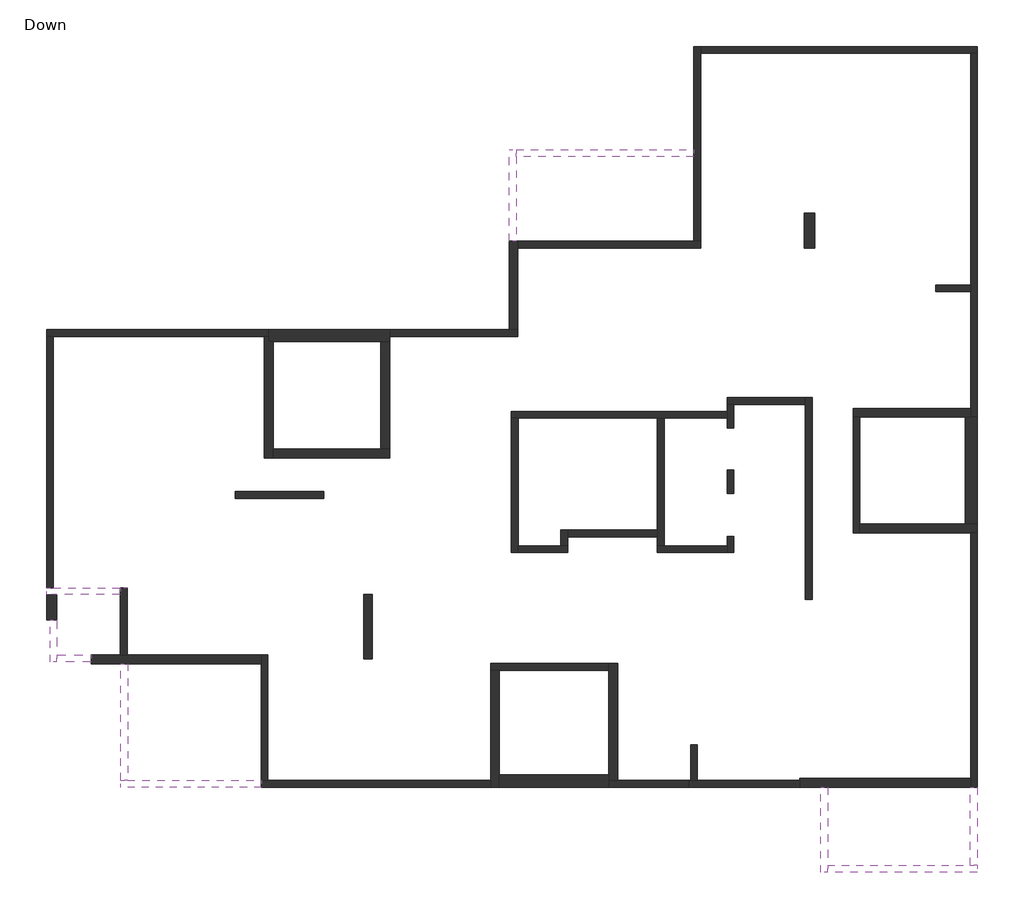
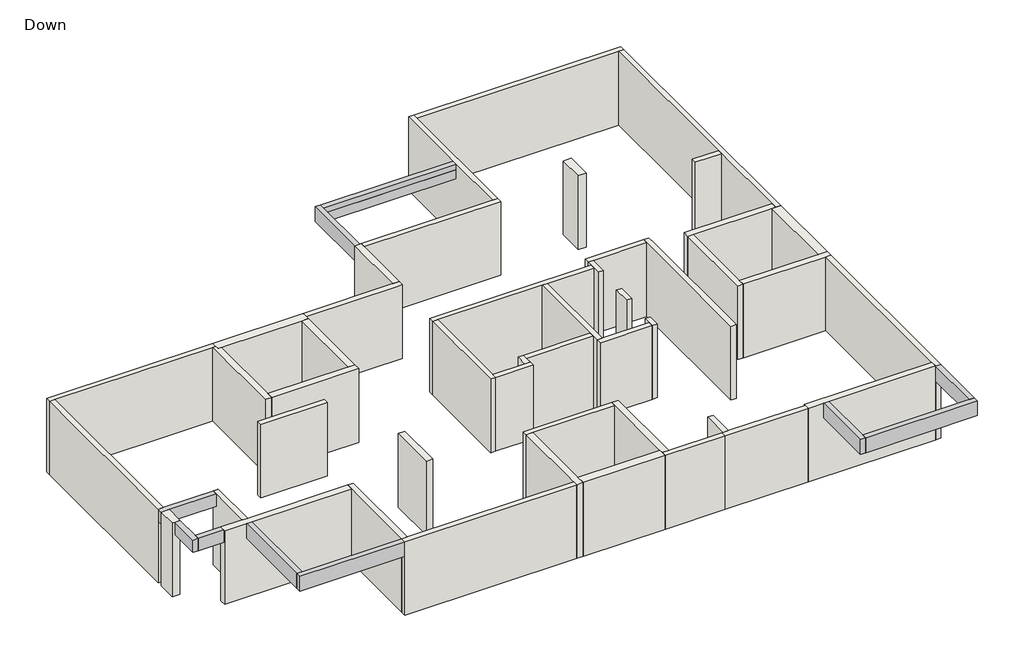
# One storey: 46 walls, 10 beams.
# Revit data of these elements (continued)
# Element 19 (IfcWall, "20") (continued)
#   SOFiSTiK_AMG_Scheduled = yes
#   SOFiSTiK_AMG_Adjusted = yes
#   Phase Created = New Construction
#   Base Constraint = Down
#   Top Constraint = Typical Floor
#   Materials on its faces: "Concrete"
# Element 20 (IfcWall, "20")
#   Comments = ""
#   Mark = "W10"
#   SOFiSTiK_EdgeZones = "W10"
#   SOFiSTiK_AMG_Comments = ""
#   Top Offset = 0 cm
#   Base Offset = 0 cm
#   wall height = 300 cm
#   SOFiSTiK_AMG_Scheduled = yes
#   SOFiSTiK_AMG_Adjusted = yes
#   Phase Created = New Construction
#   Base Constraint = Down
#   Top Constraint = Typical Floor
#   Materials on its faces: "Concrete"
# Element 21 (IfcWall, "20")
#   Comments = ""
#   Mark = "W11"
#   SOFiSTiK_EdgeZones = "W11"
#   SOFiSTiK_AMG_Comments = ""
#   Top Offset = 0 cm
#   Base Offset = 0 cm
#   wall height = 300 cm
#   SOFiSTiK_AMG_Scheduled = yes
#   SOFiSTiK_AMG_Adjusted = yes
#   Phase Created = New Construction
#   Base Constraint = Down
#   Top Constraint = Typical Floor
#   Materials on its faces: "Concrete"
# Element 22 (IfcWall, "20")
#   Comments = ""
#   Mark = "W12"
#   SOFiSTiK_EdgeZones = "W12"
#   SOFiSTiK_AMG_Comments = ""
#   Top Offset = 0 cm
#   Base Offset = 0 cm
#   wall height = 300 cm
#   SOFiSTiK_AMG_Scheduled = yes
#   SOFiSTiK_AMG_Adjusted = yes
#   Phase Created = New Construction
#   Base Constraint = Down
#   Top Constraint = Typical Floor
#   Materials on its faces: "Concrete"
# Element 23 (IfcWall, "20")
#   Comments = ""
#   Mark = "W13"
#   SOFiSTiK_EdgeZones = "W13"
#   SOFiSTiK_AMG_Comments = ""
#   Top Offset = 0 cm
#   Base Offset = 0 cm
#   wall height = 300 cm
#   SOFiSTiK_AMG_Scheduled = yes
#   SOFiSTiK_AMG_Adjusted = yes
#   Phase Created = New Construction
#   Base Constraint = Down
#   Top Constraint = Typical Floor
#   Materials on its faces: "Concrete"
# Element 24 (IfcWall, "20")
#   Comments = ""
#   Mark = "W14"
#   SOFiSTiK_EdgeZones = "W14"
#   SOFiSTiK_AMG_Comments = ""
#   Top Offset = 0 cm
#   Base Offset = 0 cm
#   wall height = 300 cm
#   SOFiSTiK_AMG_Scheduled = yes
#   SOFiSTiK_AMG_Adjusted = yes
#   Phase Created = New Construction
#   Base Constraint = Down
#   Top Constraint = Typical Floor
#   Materials on its faces: "Concrete"
# Element 25 (IfcWall, "20")
#   Comments = ""
#   Mark = "W15"
#   SOFiSTiK_EdgeZones = "W15"
#   SOFiSTiK_AMG_Comments = ""
#   Top Offset = 0 cm
#   Base Offset = 0 cm
#   wall height = 300 cm
#   SOFiSTiK_AMG_Scheduled = yes
#   SOFiSTiK_AMG_Adjusted = yes
#   Phase Created = New Construction
#   Base Constraint = Down
#   Top Constraint = Typical Floor
#   Materials on its faces: "Concrete"
# Element 26 (IfcWall, "20")
#   Comments = ""
#   Mark = "W16"
#   SOFiSTiK_EdgeZones = "W16"
#   SOFiSTiK_AMG_Comments = ""
#   Top Offset = 0 cm
#   Base Offset = 0 cm
#   wall height = 300 cm
#   SOFiSTiK_AMG_Scheduled = yes
#   SOFiSTiK_AMG_Adjusted = yes
#   Phase Created = New Construction
#   Base Constraint = Down
#   Top Constraint = Typical Floor
#   Materials on its faces: "Concrete"
# Element 27 (IfcWall, "20")
#   Comments = ""
#   Mark = "W17"
#   SOFiSTiK_EdgeZones = "W17"
#   SOFiSTiK_AMG_Comments = ""
#   Top Offset = 0 cm
#   Base Offset = 0 cm
#   wall height = 300 cm
#   SOFiSTiK_AMG_Scheduled = yes
#   SOFiSTiK_AMG_Adjusted = yes
#   Phase Created = New Construction
#   Base Constraint = Down
#   Top Constraint = Typical Floor
#   Materials on its faces: "Concrete"
# Element 28 (IfcWall, "20")
#   Comments = ""
#   Mark = "W18"
#   SOFiSTiK_EdgeZones = "W18"
#   SOFiSTiK_AMG_Comments = ""
#   Top Offset = 0 cm
#   Base Offset = 0 cm
#   wall height = 300 cm
#   SOFiSTiK_AMG_Scheduled = yes
#   SOFiSTiK_AMG_Adjusted = yes
#   Phase Created = New Construction
#   Base Constraint = Down
#   Top Constraint = Typical Floor
#   Materials on its faces: "Concrete"
# Element 29 (IfcWall, "20")
#   Comments = ""
#   Mark = "W19"
#   SOFiSTiK_EdgeZones = "W19"
#   SOFiSTiK_AMG_Comments = ""
#   Top Offset = 0 cm
#   Base Offset = 0 cm
#   wall height = 300 cm
#   SOFiSTiK_AMG_Scheduled = yes
#   SOFiSTiK_AMG_Adjusted = yes
#   Phase Created = New Construction
#   Base Constraint = Down
#   Top Constraint = Typical Floor
#   Materials on its faces: "Concrete"
# Element 30 (IfcWall, "20")
#   Comments = ""
#   Mark = "W20"
#   SOFiSTiK_EdgeZones = "W20"
#   SOFiSTiK_AMG_Comments = ""
#   Top Offset = 0 cm
#   Base Offset = 0 cm
#   wall height = 300 cm
#   SOFiSTiK_AMG_Scheduled = yes
#   SOFiSTiK_AMG_Adjusted = yes
#   Phase Created = New Construction
#   Base Constraint = Down
#   Top Constraint = Typical Floor
#   Materials on its faces: "Concrete"
# Element 31 (IfcWall, "20")
#   Comments = ""
#   Mark = "W21"
#   SOFiSTiK_EdgeZones = "W21"
#   SOFiSTiK_AMG_Comments = ""
#   Top Offset = 0 cm
#   Base Offset = 0 cm
#   wall height = 300 cm
#   SOFiSTiK_AMG_Scheduled = yes
#   SOFiSTiK_AMG_Adjusted = yes
#   Phase Created = New Construction
#   Base Constraint = Down
#   Top Constraint = Typical Floor
#   Materials on its faces: "Concrete"
# Element 32 (IfcWall, "20")
#   Comments = ""
#   Mark = "W22"
#   SOFiSTiK_EdgeZones = "W22"
#   SOFiSTiK_AMG_Comments = ""
#   Top Offset = 0 cm
#   Base Offset = 0 cm
#   wall height = 300 cm
#   SOFiSTiK_AMG_Scheduled = yes
#   SOFiSTiK_AMG_Adjusted = yes
#   Phase Created = New Construction
#   Base Constraint = Down
#   Top Constraint = Typical Floor
#   Materials on its faces: "Concrete"
# Element 33 (IfcWall, "20")
#   Comments = ""
#   Mark = "W23"
#   SOFiSTiK_EdgeZones = "W23"
#   SOFiSTiK_AMG_Comments = ""
#   Top Offset = 0 cm
#   Base Offset = 0 cm
#   wall height = 300 cm
#   SOFiSTiK_AMG_Scheduled = yes
#   SOFiSTiK_AMG_Adjusted = yes
#   Phase Created = New Construction
#   Base Constraint = Down
#   Top Constraint = Typical Floor
#   Materials on its faces: "Concrete"
# Element 34 (IfcWall, "20")
#   Comments = ""
#   Mark = "W24"
#   SOFiSTiK_EdgeZones = "W24"
#   SOFiSTiK_AMG_Comments = ""
#   Top Offset = 0 cm
#   Base Offset = 0 cm
#   wall height = 300 cm
#   SOFiSTiK_AMG_Scheduled = yes
#   SOFiSTiK_AMG_Adjusted = yes
#   Phase Created = New Construction
#   Base Constraint = Down
#   Top Constraint = Typical Floor
#   Materials on its faces: "Concrete"
# Element 35 (IfcWall, "20")
#   Comments = ""
#   Mark = "W25"
#   SOFiSTiK_EdgeZones = "W25"
#   SOFiSTiK_AMG_Comments = ""
#   Top Offset = 0 cm
#   Base Offset = 0 cm
#   wall height = 300 cm
#   SOFiSTiK_AMG_Scheduled = yes
#   SOFiSTiK_AMG_Adjusted = yes
#   Phase Created = New Construction
#   Base Constraint = Down
#   Top Constraint = Typical Floor
#   Materials on its faces: "Concrete"
# Element 36 (IfcWall, "20")
#   Comments = ""
#   Mark = "W26"
#   SOFiSTiK_EdgeZones = "W26"
#   SOFiSTiK_AMG_Comments = ""
#   Top Offset = 0 cm
#   Base Offset = 0 cm
#   wall height = 300 cm
#   SOFiSTiK_AMG_Scheduled = yes
#   SOFiSTiK_AMG_Adjusted = yes
#   Phase Created = New Construction
#   Base Constraint = Down
#   Top Constraint = Typical Floor
#   Materials on its faces: "Concrete"
# Element 37 (IfcWall, "20")
#   Comments = ""
#   Mark = "W27"
#   SOFiSTiK_EdgeZones = "W28"
#   SOFiSTiK_AMG_Comments = ""
#   Top Offset = 0 cm
#   Base Offset = 0 cm
#   wall height = 300 cm
#   SOFiSTiK_AMG_Scheduled = yes
#   SOFiSTiK_AMG_Adjusted = yes
#   Phase Created = New Construction
#   Base Constraint = Down
#   Top Constraint = Typical Floor
#   Materials on its faces: "Concrete"
# Element 38 (IfcWall, "20")
#   Comments = ""
#   Mark = "W28"
#   SOFiSTiK_EdgeZones = "W29"
#   SOFiSTiK_AMG_Comments = ""
#   Top Offset = 0 cm
#   Base Offset = 0 cm
#   wall height = 300 cm
#   SOFiSTiK_AMG_Scheduled = yes
#   SOFiSTiK_AMG_Adjusted = yes
#   Phase Created = New Construction
#   Base Constraint = Down
#   Top Constraint = Typical Floor
#   Materials on its faces: "Concrete"
# Element 39 (IfcWall, "20")
#   Comments = ""
#   Mark = "W29"
#   SOFiSTiK_EdgeZones = "W30"
#   SOFiSTiK_AMG_Comments = ""
#   Top Offset = 0 cm
#   Base Offset = 0 cm
#   wall height = 300 cm
#   SOFiSTiK_AMG_Scheduled = yes
#   SOFiSTiK_AMG_Adjusted = yes
#   Phase Created = New Construction
#   Base Constraint = Down
#   Top Constraint = Typical Floor
#   Materials on its faces: "Concrete"
# Element 40 (IfcWall, "20")
#   Comments = ""
#   Mark = "W30"
#   SOFiSTiK_EdgeZones = "W31"
#   SOFiSTiK_AMG_Comments = ""
#   Top Offset = 0 cm
#   Base Offset = 0 cm
#   wall height = 300 cm
#   SOFiSTiK_AMG_Scheduled = yes
#   SOFiSTiK_AMG_Adjusted = yes
#   Phase Created = New Construction
#   Base Constraint = Down
#   Top Constraint = Typical Floor
#   Materials on its faces: "Concrete"
# Element 41 (IfcWall, "25")
#   Comments = ""
#   Mark = "W36"
#   SOFiSTiK_EdgeZones = "W37"
#   SOFiSTiK_AMG_Comments = ""
#   Top Offset = 0 cm
#   Base Offset = 0 cm
#   wall height = 300 cm
#   SOFiSTiK_AMG_Scheduled = yes
#   SOFiSTiK_AMG_Adjusted = yes
#   Phase Created = New Construction
#   Base Constraint = Down
#   Top Constraint = Typical Floor
#   Materials on its faces: "Concrete"
# Element 42 (IfcWall, "25")
#   Comments = ""
#   Mark = "W37"
#   SOFiSTiK_EdgeZones = "W38"
#   SOFiSTiK_AMG_Comments = ""
#   Top Offset = 0 cm
#   Base Offset = 0 cm
#   wall height = 300 cm
#   SOFiSTiK_AMG_Scheduled = yes
#   SOFiSTiK_AMG_Adjusted = yes
#   Phase Created = New Construction
#   Base Constraint = Down
#   Top Constraint = Typical Floor
#   Materials on its faces: "Concrete"
# Element 43 (IfcWall, "25")
#   Comments = ""
#   Mark = "W38"
#   SOFiSTiK_EdgeZones = "W39"
#   SOFiSTiK_AMG_Comments = ""
#   Top Offset = 0 cm
#   Base Offset = 0 cm
#   wall height = 300 cm
#   SOFiSTiK_AMG_Scheduled = yes
#   SOFiSTiK_AMG_Adjusted = yes
#   Phase Created = New Construction
#   Base Constraint = Down
#   Top Constraint = Typical Floor
#   Materials on its faces: "Concrete"
# Element 44 (IfcWall, "25")
#   Comments = ""
#   Mark = "W39"
#   SOFiSTiK_EdgeZones = "W40"
#   SOFiSTiK_AMG_Comments = ""
#   Top Offset = 0 cm
#   Base Offset = 0 cm
#   wall height = 300 cm
#   SOFiSTiK_AMG_Scheduled = yes
#   SOFiSTiK_AMG_Adjusted = yes
#   Phase Created = New Construction
#   Base Constraint = Down
#   Top Constraint = Typical Floor
#   Materials on its faces: "Concrete"
# Element 45 (IfcWall, "25")
#   Comments = ""
#   Mark = "W40"
#   SOFiSTiK_EdgeZones = "W41"
#   SOFiSTiK_AMG_Comments = ""
#   Top Offset = 0 cm
#   Base Offset = 0 cm
#   wall height = 300 cm
#   SOFiSTiK_AMG_Scheduled = yes
#   SOFiSTiK_AMG_Adjusted = yes
#   Phase Created = New Construction
#   Base Constraint = Down
#   Top Constraint = Typical Floor
#   Materials on its faces: "Concrete"
# Element 46 (IfcWall, "25")
#   Comments = ""
#   Mark = "W41"
#   SOFiSTiK_EdgeZones = "W42"
#   SOFiSTiK_AMG_Comments = ""
#   Top Offset = 0 cm
#   Base Offset = 0 cm
#   wall height = 300 cm
#   SOFiSTiK_AMG_Scheduled = yes
#   SOFiSTiK_AMG_Adjusted = yes
#   Phase Created = New Construction
#   Base Constraint = Down
#   Top Constraint = Typical Floor
#   Materials on its faces: "Concrete"
# Element 47 (IfcWall, "25")
#   Comments = ""
#   Mark = "W42"
#   SOFiSTiK_EdgeZones = "W43"
#   SOFiSTiK_AMG_Comments = ""
#   Top Offset = 0 cm
#   Base Offset = 0 cm
#   wall height = 300 cm
#   SOFiSTiK_AMG_Scheduled = yes
#   SOFiSTiK_AMG_Adjusted = yes
#   Phase Created = New Construction
#   Base Constraint = Down
#   Top Constraint = Typical Floor
#   Materials on its faces: "Concrete"
# Element 48 (IfcWall, "25")
#   Comments = ""
#   Mark = "W43"
#   SOFiSTiK_EdgeZones = "W44"
#   SOFiSTiK_AMG_Comments = ""
#   Top Offset = 0 cm
#   Base Offset = 0 cm
#   wall height = 300 cm
#   SOFiSTiK_AMG_Scheduled = yes
#   SOFiSTiK_AMG_Adjusted = yes
#   Phase Created = New Construction
#   Base Constraint = Down
#   Top Constraint = Typical Floor
#   Materials on its faces: "Concrete"
# Element 49 (IfcWall, "25")
#   Comments = ""
#   Mark = "W44"
#   SOFiSTiK_EdgeZones = "W45"
#   SOFiSTiK_AMG_Comments = ""
#   Top Offset = 0 cm
#   Base Offset = 0 cm
#   wall height = 300 cm
#   SOFiSTiK_AMG_Scheduled = yes
#   SOFiSTiK_AMG_Adjusted = yes
#   Phase Created = New Construction
#   Base Constraint = Down
#   Top Constraint = Typical Floor
#   Materials on its faces: "Concrete"
# Element 50 (IfcWall, "25")
#   Comments = ""
#   Mark = "W45"
#   SOFiSTiK_EdgeZones = "W46"
#   SOFiSTiK_AMG_Comments = ""
#   Top Offset = 0 cm
#   Base Offset = 0 cm
#   wall height = 300 cm
#   SOFiSTiK_AMG_Scheduled = yes
#   SOFiSTiK_AMG_Adjusted = yes
#   Phase Created = New Construction
#   Base Constraint = Down
#   Top Constraint = Typical Floor
#   Materials on its faces: "Concrete"
# Element 51 (IfcWall, "25")
#   Comments = ""
#   Mark = "W46"
#   SOFiSTiK_EdgeZones = "W47"
#   SOFiSTiK_AMG_Comments = ""
#   Top Offset = 0 cm
#   Base Offset = 0 cm
#   wall height = 300 cm
#   SOFiSTiK_AMG_Scheduled = yes
#   SOFiSTiK_AMG_Adjusted = yes
#   Phase Created = New Construction
#   Base Constraint = Down
#   Top Constraint = Typical Floor
#   Materials on its faces: "Concrete"
# Element 52 (IfcWall, "30")
#   Comments = ""
#   Mark = "W31"
#   SOFiSTiK_EdgeZones = "W32"
#   SOFiSTiK_AMG_Comments = ""
#   Top Offset = 0 cm
#   Base Offset = 0 cm
#   wall height = 300 cm
#   SOFiSTiK_AMG_Scheduled = yes
#   SOFiSTiK_AMG_Adjusted = yes
#   Phase Created = New Construction
#   Base Constraint = Down
#   Top Constraint = Typical Floor
#   Materials on its faces: "Concrete"
# Element 53 (IfcWall, "30")
#   Comments = ""
#   Mark = "W32"
#   SOFiSTiK_EdgeZones = "W33"
#   SOFiSTiK_AMG_Comments = ""
#   Top Offset = 0 cm
#   Base Offset = 0 cm
#   wall height = 300 cm
#   SOFiSTiK_AMG_Scheduled = yes
#   SOFiSTiK_AMG_Adjusted = yes
#   Phase Created = New Construction
#   Base Constraint = Down
#   Top Constraint = Typical Floor
#   Materials on its faces: "Concrete"
# Element 54 (IfcWall, "35")
#   Comments = ""
#   Mark = "W33"
#   SOFiSTiK_EdgeZones = "W34"
#   SOFiSTiK_AMG_Comments = ""
#   Top Offset = 0 cm
#   Base Offset = 0 cm
#   wall height = 300 cm
#   SOFiSTiK_AMG_Scheduled = yes
#   SOFiSTiK_AMG_Adjusted = yes
#   Phase Created = New Construction
#   Base Constraint = Down
#   Top Constraint = Typical Floor
#   Materials on its faces: "Concrete"
# Element 55 (IfcWall, "35")
#   Comments = ""
#   Mark = "W34"
#   SOFiSTiK_EdgeZones = "W35"
#   SOFiSTiK_AMG_Comments = ""
#   Top Offset = 0 cm
#   Base Offset = 0 cm
#   wall height = 300 cm
#   SOFiSTiK_AMG_Scheduled = yes
#   SOFiSTiK_AMG_Adjusted = yes
#   Phase Created = New Construction
#   Base Constraint = Down
#   Top Constraint = Typical Floor
#   Materials on its faces: "Concrete"
# Element 56 (IfcWall, "35")
#   Comments = ""
#   Mark = "W35"
#   SOFiSTiK_EdgeZones = "W36"
#   SOFiSTiK_AMG_Comments = ""
#   Top Offset = 0 cm
#   Base Offset = 0 cm
#   wall height = 300 cm
#   SOFiSTiK_AMG_Scheduled = yes
#   SOFiSTiK_AMG_Adjusted = yes
#   Phase Created = New Construction
#   Base Constraint = Down
#   Top Constraint = Typical Floor
#   Materials on its faces: "Concrete"
# Materials
#   "Concrete": class "Concrete", colour RGB 192 192 192, transparency 0, Keynote = "01000", Description = "Cast-in-place concrete", Cost = 0
